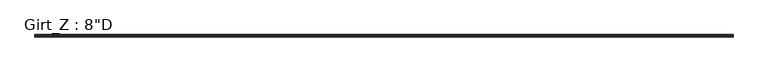
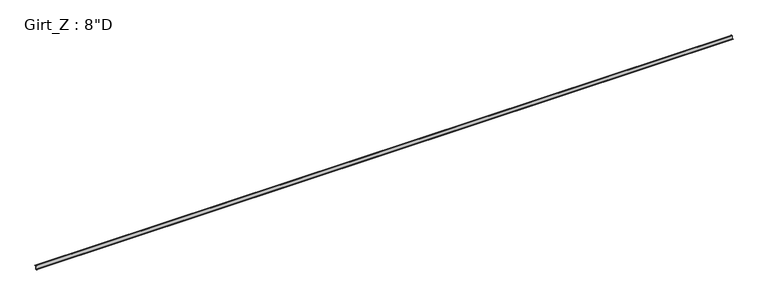
"""IFC4 building model written with IfcOpenShell, lengths in millimetres: beam geometry."""

from ifc_helpers import new_model, si_unit, point, frame, frame_2d, origin, place, context, project, spatial, polyline, circle_curve, trimmed, segment, composite_curve, outline, extrude, source, transform, mapped, element, save


def beam_732a92f4(model_context):
    return source(origin(), model_context, "Body", "SweptSolid", [
        extrude(outline(composite_curve([segment(polyline([(63.5, 101.6), (75.745104, 87.0068534), (73.6169367, 85.221109), (62.204539, 98.821875), (3.3005807, 98.821875)]), True, "CONTINUOUS"), segment(trimmed(circle_curve(frame_2d((3.3741066, 96.8381931)), 1.9850441), [point((3.3005807, 98.821875))], [point((1.3890625, 96.8381931))], True, "CARTESIAN"), True, "CONTINUOUS"), segment(polyline([(1.3890625, 96.8381931), (1.3890625, -96.8375)]), True, "CONTINUOUS"), segment(trimmed(circle_curve(frame_2d((-3.3734375, -96.8375)), 4.7625), [point((1.3890625, -96.8375))], [point((-3.3734375, -101.6))], False, "CARTESIAN"), True, "CONTINUOUS"), segment(polyline([(-3.3734375, -101.6), (-63.5, -101.6), (-75.745104, -87.0068534), (-73.6169367, -85.221109), (-62.204539, -98.821875), (-3.2694106, -98.821875)]), True, "CONTINUOUS"), segment(trimmed(circle_curve(frame_2d((-3.3748024, -96.8389339)), 1.9857399), [point((-3.2694106, -98.821875))], [point((-1.3890625, -96.8389339))], True, "CARTESIAN"), True, "CONTINUOUS"), segment(polyline([(-1.3890625, -96.8389339), (-1.3890625, 96.8375)]), True, "CONTINUOUS"), segment(trimmed(circle_curve(frame_2d((3.3734375, 96.8375)), 4.7625), [point((-1.3890625, 96.8375))], [point((3.3734375, 101.6))], False, "CARTESIAN"), True, "CONTINUOUS"), segment(polyline([(3.3734375, 101.6), (63.5, 101.6)]), True, "CONTINUOUS")], self_intersect=False)), frame((-20834.35, 0.0, 0.0), z_axis=(1.0, 0.0, 0.0), x_axis=(0.0, 1.0, 0.0)), (0.0, 0.0, 1.0), 41636.95),
    ])


if __name__ == "__main__":
    model = new_model("IFC4")
    model_context = context("Model", 3, world=origin())
    ifc_project = project(units=[si_unit("LENGTHUNIT", "METRE", prefix="MILLI")], contexts=[model_context])
    site = spatial("IfcSite", under=ifc_project)
    building = spatial("IfcBuilding", under=site)
    placement = place(None, origin())
    beam_shape = beam_732a92f4(model_context)
    element("IfcBeam", 1, ObjectType="Girt_Z : 8\"D", at=placement, inside=building, context=model_context, shape_type="MappedRepresentation", body=[
        mapped(beam_shape, transform((0.0, 0.0, 0.0), x_axis=(1.0, 0.0, 0.0), y_axis=(0.0, 1.0, 0.0), z_axis=(0.0, 0.0, 1.0))),
    ])
    save(model, "model.ifc")

# Revit data of these elements
# Type "Girt_Z : 8\"D"
#   Web_Thickness = 0' - 0 7/64"
#   Length [instance default] = 10' - 0"
#   Leg_1 = 0' - 2 1/2"
#   Height = 0' - 8"
#   Structural Material [instance default] = none
